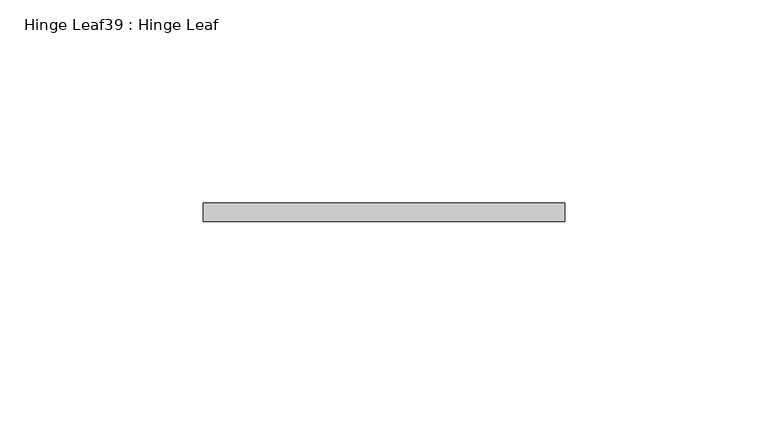
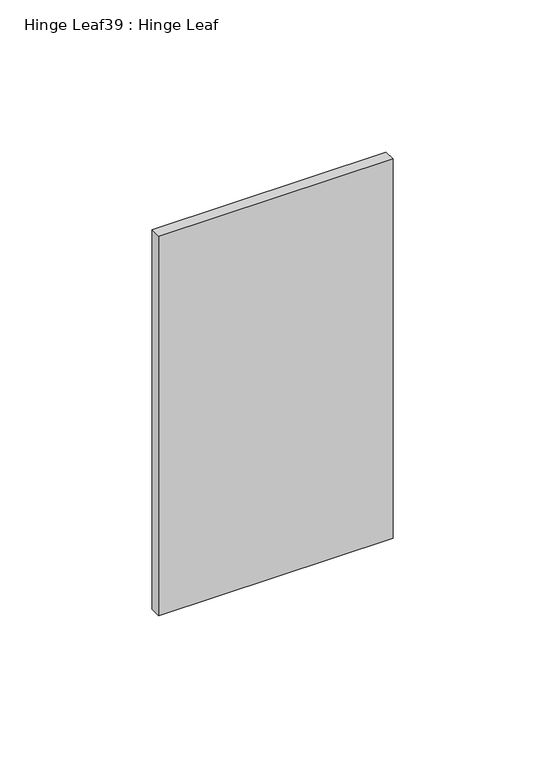
"""IFC4 building model written with IfcOpenShell, lengths in millimetres: proxy geometry, Hinge Leaf39 : Hinge Leaf."""

from ifc_helpers import new_model, si_unit, frame, origin, place, context, project, spatial, polyline, outline, extrude, source, transform, mapped, element, save


def hinge_leaf39_hinge_leaf_b84fefac(model_context):
    return source(origin(), model_context, "Body", "SweptSolid", [
        extrude(outline(polyline([(587327.7934739, -534096.6663841), (587416.6934739, -534096.6663841), (587416.6934739, -534101.2383841), (587327.7934739, -534101.2383841), (587327.7934739, -534096.6663841)])), frame((0.0, 0.0, 311.15), z_axis=(0.0, 0.0, 1.0), x_axis=(1.0, 0.0, 0.0)), (0.0, 0.0, 1.0), 152.4),
    ])


if __name__ == "__main__":
    model = new_model("IFC4")
    model_context = context("Model", 3, world=origin())
    ifc_project = project(units=[si_unit("LENGTHUNIT", "METRE", prefix="MILLI")], contexts=[model_context])
    site = spatial("IfcSite", under=ifc_project)
    building = spatial("IfcBuilding", under=site)
    placement = place(None, origin())
    hinge_leaf39_hinge_leaf_shape = hinge_leaf39_hinge_leaf_b84fefac(model_context)
    element("IfcBuildingElementProxy", 1, Name="Hinge Leaf39 : Hinge Leaf", ObjectType="Hinge Leaf39 : Hinge Leaf", at=placement, inside=building, context=model_context, shape_type="MappedRepresentation", body=[
        mapped(hinge_leaf39_hinge_leaf_shape, transform((0.0, 0.0, 0.0), x_axis=(1.0, 0.0, 0.0), y_axis=(0.0, 1.0, 0.0), z_axis=(0.0, 0.0, 1.0))),
    ])
    save(model, "model.ifc")

# Revit data of these elements
# Element 1 (IfcBuildingElementProxy, "Hinge Leaf39 : Hinge Leaf")
#   Materials on its faces: "6\"X6\" WELD-ON STL BUTT HINGE"
# Materials
#   "6\"X6\" WELD-ON STL BUTT HINGE": class "Metal", colour RGB 189 187 185, transparency 0, Description = "Carbon steel", Cost = 0
